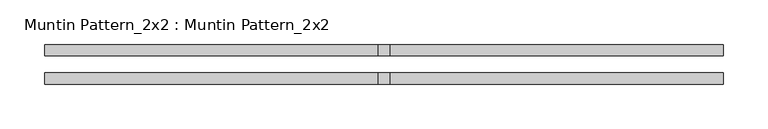
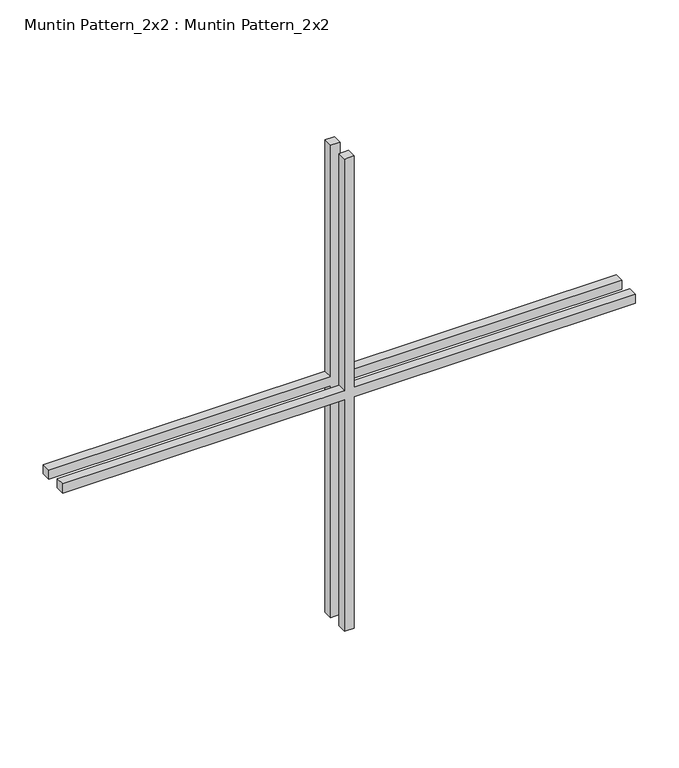
"""IFC4 building model written with IfcOpenShell, lengths in millimetres: proxy geometry, Muntin Pattern_2x2 : Muntin Pattern_2x2."""

from ifc_helpers import new_model, si_unit, frame, origin, place, context, project, spatial, polyline, outline, extrude, source, transform, mapped, element, save


def muntin_pattern_2x2_muntin_pattern_2x2_8646dbc3(model_context):
    return source(origin(), model_context, "Body", "SweptSolid", [
        extrude(outline(polyline([(338.1375, -6.35), (338.1375, -381.0), (325.4375, -381.0), (325.4375, -6.35), (0.0, -6.35), (0.0, 6.35), (325.4375, 6.35), (325.4375, 381.0), (338.1375, 381.0), (338.1375, 6.35), (663.575, 6.35), (663.575, -6.35), (338.1375, -6.35)])), frame((0.0, 9.525, 0.0), z_axis=(0.0, 1.0, 0.0), x_axis=(0.0, 0.0, 1.0)), (0.0, 0.0, 1.0), 12.7),
        extrude(outline(polyline([(338.1375, -6.35), (338.1375, -381.0), (325.4375, -381.0), (325.4375, -6.35), (0.0, -6.35), (0.0, 6.35), (325.4375, 6.35), (325.4375, 381.0), (338.1375, 381.0), (338.1375, 6.35), (663.575, 6.35), (663.575, -6.35), (338.1375, -6.35)])), frame((0.0, -22.225, 0.0), z_axis=(0.0, 1.0, 0.0), x_axis=(0.0, 0.0, 1.0)), (0.0, 0.0, 1.0), 12.7),
    ])


if __name__ == "__main__":
    model = new_model("IFC4")
    model_context = context("Model", 3, world=origin())
    ifc_project = project(units=[si_unit("LENGTHUNIT", "METRE", prefix="MILLI")], contexts=[model_context])
    site = spatial("IfcSite", under=ifc_project)
    building = spatial("IfcBuilding", under=site)
    placement = place(None, origin())
    muntin_pattern_2x2_muntin_pattern_2x2_shape = muntin_pattern_2x2_muntin_pattern_2x2_8646dbc3(model_context)
    element("IfcBuildingElementProxy", 1, Name="Muntin Pattern_2x2 : Muntin Pattern_2x2", ObjectType="Muntin Pattern_2x2 : Muntin Pattern_2x2", at=placement, inside=building, context=model_context, shape_type="MappedRepresentation", body=[
        mapped(muntin_pattern_2x2_muntin_pattern_2x2_shape, transform((0.0, 0.0, 0.0), x_axis=(1.0, 0.0, 0.0), y_axis=(0.0, 1.0, 0.0), z_axis=(0.0, 0.0, 1.0))),
    ])
    save(model, "model.ifc")

# Revit data of these elements
# Type "Muntin Pattern_2x2 : Muntin Pattern_2x2"
#   Width [instance default] = 4' - 0"
#   Thickness = 0' - 0 1/2"
#   Height [instance default] = 4' - 0"
#   Distance = 0' - 0 3/4"
#   Interior Material [instance default] = none
#   Exterior Material [instance default] = none
#   Default Elevation = 0
# Element 1 (IfcBuildingElementProxy, "Muntin Pattern_2x2 : Muntin Pattern_2x2")
#   Width = 2' - 6"
#   Height = 2' - 2 1/8"
#   Interior Material = Wood - Stained
#   Exterior Material = Clad - White
#   Materials on its faces: "Clad - White", "Wood - Stained"
# Materials
#   "Clad - White": class "Wood", colour RGB 242 242 238, transparency 0, Cost = 0
#   "Wood - Stained": class "Wood", colour RGB 224 178 126, transparency 0, Cost = 0
